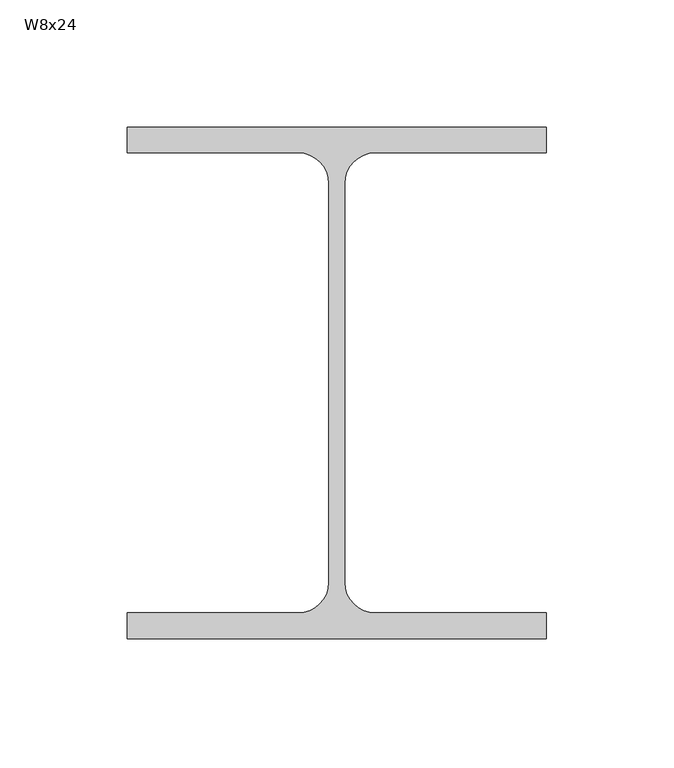
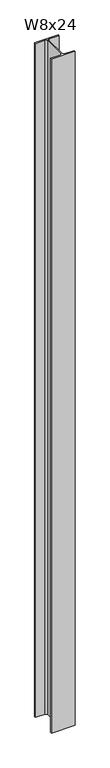
"""IFC4 building model written with IfcOpenShell, lengths in millimetres: column geometry, RME WF - Column : W8x24."""

import ifcopenshell
import ifcopenshell.guid

model = None  # the IFC model being written
_history = None  # IfcOwnerHistory: only IFC2X3 demands one
_inside = {}  # id of a spatial element -> (the spatial element, [elements in it])
_under = {}  # id of a project, library or spatial element -> (it, [spatial elements below it])
_declared = {}  # id of a project -> (the project, [libraries it declares])
_typed = {}  # id of a type object -> (the type object, [elements of that type])
_made_of = {}  # id of a material, layer set ... -> (it, [elements and type objects made of it])


def new_model(schema):
    """Start an empty IFC model of exactly this schema.

    Asked for "IFC4X3", IfcOpenShell would pick the latest addendum, in which some entities
    have other attributes; the version numbers below select the first issue.
    IFC2X3 requires an IfcOwnerHistory on every rooted entity: one is made here for all.
    """
    global model, _history
    if schema == "IFC4X3":
        model = ifcopenshell.file(schema_version=(4, 3, 0, 0))
    else:
        model = ifcopenshell.file(schema=schema)
    _inside.clear()
    _under.clear()
    _declared.clear()
    _typed.clear()
    _made_of.clear()
    _history = None
    if model.schema == "IFC2X3":
        org = make("IfcOrganization", Name="unknown")
        user = make(
            "IfcPersonAndOrganization",
            ThePerson=make("IfcPerson", FamilyName="unknown"),
            TheOrganization=org,
        )
        app = make(
            "IfcApplication",
            ApplicationDeveloper=org,
            Version="unknown",
            ApplicationFullName="unknown",
            ApplicationIdentifier="unknown",
        )
        _history = make(
            "IfcOwnerHistory",
            OwningUser=user,
            OwningApplication=app,
            ChangeAction="ADDED",
            CreationDate=0,
        )
    return model


def make(cls, **values):
    """One entity of the class cls with the attributes given. An attribute that is None is left unset."""
    return model.create_entity(
        cls, **{name: value for name, value in values.items() if value is not None}
    )


def rooted(cls, **values):
    """An entity with a GlobalId (a new one), such as an element, a storey or a relation."""
    return make(cls, GlobalId=ifcopenshell.guid.new(), OwnerHistory=_history, **values)


def si_unit(unit_type, name, prefix=None):
    """IfcSIUnit, for example si_unit("LENGTHUNIT", "METRE", prefix="MILLI")."""
    return make("IfcSIUnit", UnitType=unit_type, Prefix=prefix, Name=name)


def assignment(units):
    """IfcUnitAssignment: the units of a project."""
    return None if units is None else make("IfcUnitAssignment", Units=units)


def point(xyz):
    """IfcCartesianPoint."""
    return None if xyz is None else make("IfcCartesianPoint", Coordinates=xyz)


def direction(xyz):
    """IfcDirection."""
    return None if xyz is None else make("IfcDirection", DirectionRatios=xyz)


def frame(location, z_axis=None, x_axis=None):
    """IfcAxis2Placement3D, a coordinate frame: its origin and axes. An axis left out is left unset."""
    return make(
        "IfcAxis2Placement3D",
        Location=point(location),
        Axis=direction(z_axis),
        RefDirection=direction(x_axis),
    )


def frame_2d(location, x_axis=None):
    """IfcAxis2Placement2D, a coordinate frame in the plane: its origin and x axis."""
    return make(
        "IfcAxis2Placement2D", Location=point(location), RefDirection=direction(x_axis)
    )


def origin():
    """The frame at (0, 0, 0) with its axes left unset."""
    return frame((0.0, 0.0, 0.0))


def place(relative_to, where):
    """IfcLocalPlacement: puts the frame where relative to a parent placement (None: the world)."""
    return make(
        "IfcLocalPlacement", PlacementRelTo=relative_to, RelativePlacement=where
    )


def context(
    kind, dimensions, precision=None, world=None, true_north=None, identifier=None
):
    """IfcGeometricRepresentationContext, for example the 3D "Model" context."""
    return make(
        "IfcGeometricRepresentationContext",
        ContextIdentifier=identifier,
        ContextType=kind,
        CoordinateSpaceDimension=dimensions,
        Precision=precision,
        WorldCoordinateSystem=world,
        TrueNorth=true_north,
    )


def project(units=None, contexts=None):
    """IfcProject with its units and contexts."""
    return rooted(
        "IfcProject",
        Name="project",
        RepresentationContexts=contexts,
        UnitsInContext=assignment(units),
    )


def spatial(cls, under=None, at=None, **own):
    """A site, building, storey or space (cls), placed at a placement, below another one or the project."""
    s = rooted(cls, ObjectPlacement=at, **own)
    if under is not None:
        _under.setdefault(under.id(), (under, []))[1].append(s)
    return s


def polyline(points):
    """IfcPolyline through the points."""
    return make("IfcPolyline", Points=[point(p) for p in points])


def circle_curve(where, radius):
    """IfcCircle in the frame where."""
    return make("IfcCircle", Position=where, Radius=radius)


def trimmed(basis, trim1, trim2, sense, master):
    """IfcTrimmedCurve: the piece of a basis curve between two trims."""
    return make(
        "IfcTrimmedCurve",
        BasisCurve=basis,
        Trim1=trim1,
        Trim2=trim2,
        SenseAgreement=sense,
        MasterRepresentation=master,
    )


def segment(curve, same_sense, transition):
    """IfcCompositeCurveSegment."""
    return make(
        "IfcCompositeCurveSegment",
        Transition=transition,
        SameSense=same_sense,
        ParentCurve=curve,
    )


def composite_curve(segments, self_intersect=None):
    """IfcCompositeCurve: segments joined end to end."""
    return make("IfcCompositeCurve", Segments=segments, SelfIntersect=self_intersect)


def outline(outer, holes=None, kind="AREA"):
    """IfcArbitraryClosedProfileDef: a profile drawn as a closed curve; with holes, ...WithVoids."""
    if holes is None:
        return make("IfcArbitraryClosedProfileDef", ProfileType=kind, OuterCurve=outer)
    return make(
        "IfcArbitraryProfileDefWithVoids",
        ProfileType=kind,
        OuterCurve=outer,
        InnerCurves=holes,
    )


def extrude(swept, where, along, depth):
    """IfcExtrudedAreaSolid: the profile swept, set in the frame where, extruded along a direction by depth."""
    return make(
        "IfcExtrudedAreaSolid",
        SweptArea=swept,
        Position=where,
        ExtrudedDirection=direction(along),
        Depth=depth,
    )


def shape(context_of_items, identifier, shape_type, items):
    """IfcShapeRepresentation: the items that make up one representation, for example the "Body"."""
    return make(
        "IfcShapeRepresentation",
        ContextOfItems=context_of_items,
        RepresentationIdentifier=identifier,
        RepresentationType=shape_type,
        Items=items,
    )


def source(mapping_origin, context_of_items, identifier, shape_type, items):
    """IfcRepresentationMap: a shape defined once, which mapped items show again and again."""
    return make(
        "IfcRepresentationMap",
        MappingOrigin=mapping_origin,
        MappedRepresentation=shape(context_of_items, identifier, shape_type, items),
    )


def transform(
    local_origin,
    x_axis=None,
    y_axis=None,
    z_axis=None,
    scale=None,
    scale2=None,
    scale3=None,
    uniform=True,
):
    """IfcCartesianTransformationOperator3D, or its non-uniform kind. x_axis, y_axis, z_axis: its Axis1, 2, 3."""
    if uniform:
        return make(
            "IfcCartesianTransformationOperator3D",
            Axis1=direction(x_axis),
            Axis2=direction(y_axis),
            LocalOrigin=point(local_origin),
            Scale=scale,
            Axis3=direction(z_axis),
        )
    return make(
        "IfcCartesianTransformationOperator3DnonUniform",
        Axis1=direction(x_axis),
        Axis2=direction(y_axis),
        LocalOrigin=point(local_origin),
        Scale=scale,
        Axis3=direction(z_axis),
        Scale2=scale2,
        Scale3=scale3,
    )


def mapped(mapping_source, mapping_target):
    """IfcMappedItem: shows the shape of a source again, moved by a transform."""
    return make(
        "IfcMappedItem", MappingSource=mapping_source, MappingTarget=mapping_target
    )


def made_of(thing, what):
    """Note that an element or type object is made of a material, layer set ...; save() writes the relation."""
    if what is not None:
        _made_of.setdefault(what.id(), (what, []))[1].append(thing)
    return thing


def element(
    cls,
    number,
    at=None,
    inside=None,
    cuts=None,
    type_object=None,
    material=None,
    context=None,
    identifier="Body",
    shape_type=None,
    held_by="IfcProductDefinitionShape",
    body=None,
    shapes=None,
    **own,
):
    """One element of the class cls, such as IfcWall. Its Tag is "e" and its number.

    at: its placement. inside: the storey or other place that contains it. cuts: it is an
    opening in that element (IfcRelVoidsElement). A single representation is given by context,
    identifier, shape_type and body (its items); several are given by shapes. held_by: the class
    of the entity that holds the representations. save() writes the other relations.
    """
    e = rooted(cls, Tag="e%d" % number, ObjectPlacement=at, **own)
    if body is not None:
        shapes = [shape(context, identifier, shape_type, body)]
    if shapes is not None:
        e.Representation = make(held_by, Representations=shapes)
    if inside is not None:
        _inside.setdefault(inside.id(), (inside, []))[1].append(e)
    if cuts is not None:
        rooted(
            "IfcRelVoidsElement", RelatingBuildingElement=cuts, RelatedOpeningElement=e
        )
    if type_object is not None:
        _typed.setdefault(type_object.id(), (type_object, []))[1].append(e)
    return made_of(e, material)


def aggregate(whole, parts):
    """IfcRelAggregates: a whole, such as a stair, and the parts it consists of."""
    return rooted("IfcRelAggregates", RelatingObject=whole, RelatedObjects=parts)


def save(model, path):
    """Write the relations noted so far, then the file.

    IfcRelAggregates (storeys below a building ...), IfcRelContainedInSpatialStructure (elements
    in a storey), IfcRelDefinesByType, IfcRelAssociatesMaterial and IfcRelDeclares: one each for
    every whole, place, type object, material and project.
    """
    for whole, parts in _under.values():
        aggregate(whole, parts)
    for where, things in _inside.values():
        rooted(
            "IfcRelContainedInSpatialStructure",
            RelatedElements=things,
            RelatingStructure=where,
        )
    for kind, things in _typed.values():
        rooted("IfcRelDefinesByType", RelatedObjects=things, RelatingType=kind)
    for what, things in _made_of.values():
        rooted("IfcRelAssociatesMaterial", RelatedObjects=things, RelatingMaterial=what)
    for by, libraries in _declared.values():
        rooted("IfcRelDeclares", RelatingContext=by, RelatedDefinitions=libraries)
    model.write(path)


def w8x24_fabf0e6b(model_context):
    return source(origin(), model_context, "Body", "SweptSolid", [
        extrude(outline(composite_curve([segment(polyline([(82.55, 100.711), (82.55, 90.551), (15.1765, 90.551)]), True, "CONTINUOUS"), segment(trimmed(circle_curve(frame_2d((15.1765, 78.486)), 12.065), [point((15.1765, 90.551))], [point((3.1115, 78.486))], True, "CARTESIAN"), True, "CONTINUOUS"), segment(polyline([(3.1115, 78.486), (3.1115, -78.486)]), True, "CONTINUOUS"), segment(trimmed(circle_curve(frame_2d((15.1765, -78.486)), 12.065), [point((3.1115, -78.486))], [point((15.1765, -90.551))], True, "CARTESIAN"), True, "CONTINUOUS"), segment(polyline([(15.1765, -90.551), (82.55, -90.551), (82.55, -100.711), (-82.55, -100.711), (-82.55, -90.551), (-15.1765, -90.551)]), True, "CONTINUOUS"), segment(trimmed(circle_curve(frame_2d((-15.1765, -78.486)), 12.065), [point((-15.1765, -90.551))], [point((-3.1115, -78.486))], True, "CARTESIAN"), True, "CONTINUOUS"), segment(polyline([(-3.1115, -78.486), (-3.1115, 78.486)]), True, "CONTINUOUS"), segment(trimmed(circle_curve(frame_2d((-15.1765, 78.486)), 12.065), [point((-3.1115, 78.486))], [point((-15.1765, 90.551))], True, "CARTESIAN"), True, "CONTINUOUS"), segment(polyline([(-15.1765, 90.551), (-82.55, 90.551), (-82.55, 100.711), (82.55, 100.711)]), True, "CONTINUOUS")], self_intersect=False)), frame((0.0, 0.0, -304.8), z_axis=(0.0, 0.0, 1.0), x_axis=(1.0, 0.0, 0.0)), (0.0, 0.0, 1.0), 4965.7),
    ])


if __name__ == "__main__":
    model = new_model("IFC4")
    model_context = context("Model", 3, world=origin())
    ifc_project = project(units=[si_unit("LENGTHUNIT", "METRE", prefix="MILLI")], contexts=[model_context])
    site = spatial("IfcSite", under=ifc_project)
    building = spatial("IfcBuilding", under=site)
    placement = place(None, origin())
    w8x24_shape = w8x24_fabf0e6b(model_context)
    element("IfcColumn", 1, ObjectType="RME WF - Column : W8x24", at=placement, inside=building, context=model_context, shape_type="MappedRepresentation", body=[
        mapped(w8x24_shape, transform((0.0, 0.0, 0.0), x_axis=(1.0, 0.0, 0.0), y_axis=(0.0, 1.0, 0.0), z_axis=(0.0, 0.0, 1.0))),
    ])
    save(model, "model.ifc")

# Revit data of these elements
# Type "RME WF - Column : W8x24"
#   Type Mark = "C1"
#   REINF TYPE [instance default] = ""
#   Nominal Size = "W16"
#   COL REMARKS [instance default] = ""
#   BP [instance default] = ""
#   Assembly Code = "B10"
#   W = 24
#   bf = 0' - 6 1/2"
#   d = 0' - 7.93"
#   k = 0' - 0 7/8"
#   kr = 0' - 0.475"
#   tf = 0' - 0.4"
#   tw = 0' - 0.245"
#   A = 0.0491667 SF
#   Structural Material [instance default] = Metal - Steel - ASTM A992
# Element 1 (IfcColumn, "RME WF - Column : W8x24")
#   Materials on its faces: "Metal - Steel - ASTM A992"
# Materials
#   "Metal - Steel - ASTM A992": class "Metal", colour RGB 255 128 0, transparency 0
